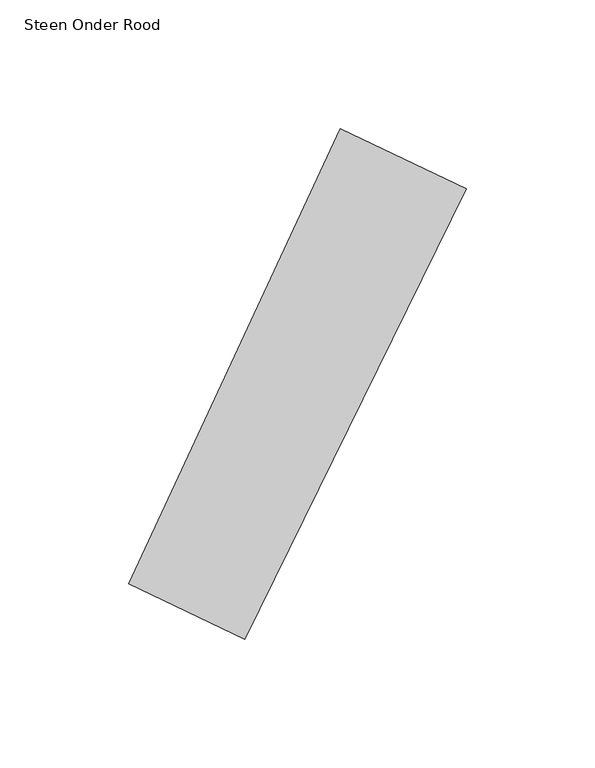
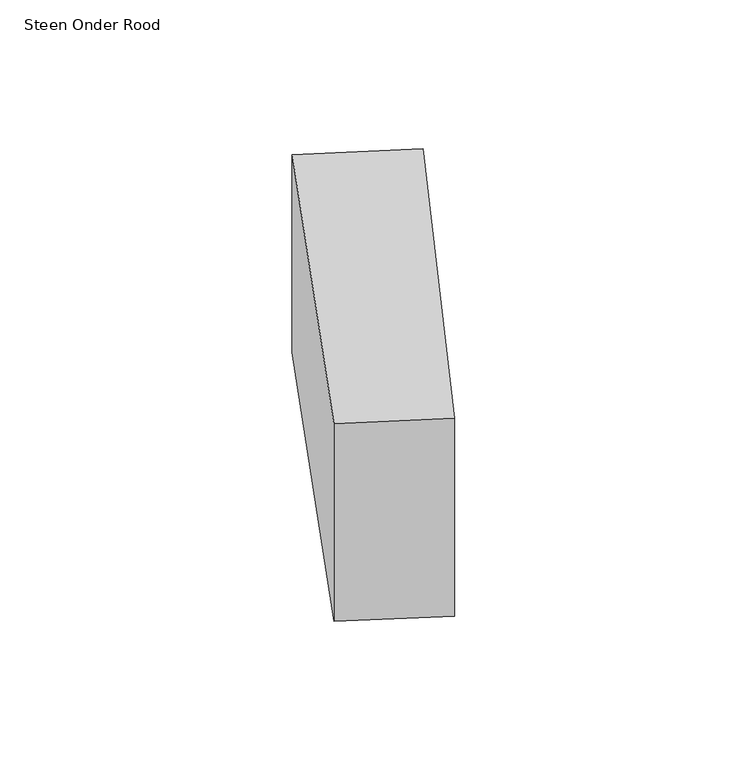
"""IFC4 building model written with IfcOpenShell, lengths in millimetres: proxy geometry, 00_GMA_steen_versie_4 : Steen Onder Rood."""

from ifc_helpers import new_model, si_unit, origin, origin_with_axes, place, context, project, spatial, polyline, outline, extrude, source, transform, mapped, element, save


def steen_onder_rood_07c1b291(model_context):
    return source(origin(), model_context, "Body", "SweptSolid", [
        extrude(outline(polyline([(142.9703865, 156.0066307), (56.9072973, -18.9875392), (11.7974439, 2.578664), (93.9510062, 179.4419078), (142.9703865, 156.0066307)])), origin_with_axes(), (0.0, 0.0, 1.0), 100.0),
    ])


if __name__ == "__main__":
    model = new_model("IFC4")
    model_context = context("Model", 3, world=origin())
    ifc_project = project(units=[si_unit("LENGTHUNIT", "METRE", prefix="MILLI")], contexts=[model_context])
    site = spatial("IfcSite", under=ifc_project)
    building = spatial("IfcBuilding", under=site)
    placement = place(None, origin())
    steen_onder_rood_shape = steen_onder_rood_07c1b291(model_context)
    element("IfcBuildingElementProxy", 1, Name="00_GMA_steen_versie_4 : Steen Onder Rood", ObjectType="00_GMA_steen_versie_4 : Steen Onder Rood", at=placement, inside=building, context=model_context, shape_type="MappedRepresentation", body=[
        mapped(steen_onder_rood_shape, transform((0.0, 0.0, 0.0), x_axis=(1.0, 0.0, 0.0), y_axis=(0.0, 1.0, 0.0), z_axis=(0.0, 0.0, 1.0))),
    ])
    save(model, "model.ifc")

# Revit data of these elements
# Type "00_GMA_steen_versie_4 : Steen Onder Rood"
#   StootVoegHalfBoven [instance default] = 5 mm
#   StootVoegHalf [instance default] = 5 mm
#   StootVoegBreedteOnder = 10 mm
#   StootVoegBreedteBoven = 10 mm
#   Steendikte = 100 mm
#   LintVoegOnderHalf = 0 mm
#   LintVoegOnder = 0 mm
#   LintVoegBovenHalf = 5 mm
#   LintVoegBoven = 10 mm
#   materiaal = 21_steen_rood
#   MateriaalVoeg = none
#   Default Elevation = 0
# Element 1 (IfcBuildingElementProxy, "00_GMA_steen_versie_4 : Steen Onder Rood")
#   Materials on its faces: "21_steen_rood"
# Materials
#   "21_steen_rood": class "Unassigned", colour RGB 213 111 43, transparency 0, Cost = 0
